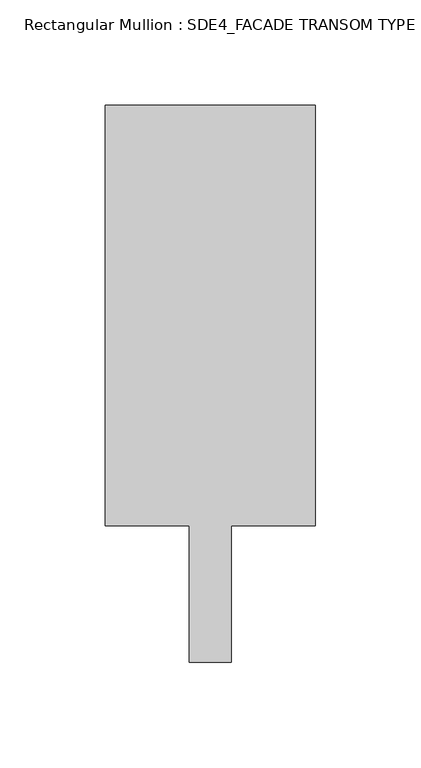
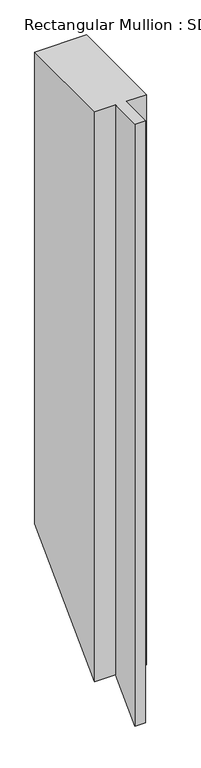
"""IFC4 building model written with IfcOpenShell, lengths in millimetres: member geometry, Rectangular Mullion : SDE4_FACADE TRANSOM TYPE 2."""

from ifc_helpers import new_model, si_unit, origin, place, context, project, spatial, faceted_brep, source, transform, mapped, element, save


def rectangular_mullion_sde4_facade_transom_type_2_6ebeb50c(model_context):
    return source(origin(), model_context, "Body", "Brep", [
        faceted_brep([(50.0, 132.5, 0.0), (-50.0, 132.5, 0.0), (-50.0, -67.5, 0.0), (-10.0, -67.5, 0.0), (-10.0, -132.5, 0.0), (10.0, -132.5, 0.0), (10.0, -67.5, 0.0), (50.0, -67.5, 0.0), (50.0, 132.5, -960.0), (-50.0, 132.5, -960.0), (-50.0, -67.5, -1160.0), (-10.0, -67.5, -1160.0), (-10.0, -132.5, -1225.0), (10.0, -132.5, -1225.0), (10.0, -67.5, -1160.0), (50.0, -67.5, -1160.0)], [[[0, 1, 2, 3, 4, 5, 6, 7]], [[1, 0, 8, 9]], [[2, 1, 9, 10]], [[3, 2, 10, 11]], [[4, 3, 11, 12]], [[5, 4, 12, 13]], [[6, 5, 13, 14]], [[7, 6, 14, 15]], [[0, 7, 15, 8]], [[8, 15, 14, 13, 12, 11, 10, 9]]]),
    ])


if __name__ == "__main__":
    model = new_model("IFC4")
    model_context = context("Model", 3, world=origin())
    ifc_project = project(units=[si_unit("LENGTHUNIT", "METRE", prefix="MILLI")], contexts=[model_context])
    site = spatial("IfcSite", under=ifc_project)
    building = spatial("IfcBuilding", under=site)
    placement = place(None, origin())
    rectangular_mullion_sde4_facade_transom_type_2_shape = rectangular_mullion_sde4_facade_transom_type_2_6ebeb50c(model_context)
    element("IfcMember", 1, ObjectType="Rectangular Mullion : SDE4_FACADE TRANSOM TYPE 2", at=placement, inside=building, context=model_context, shape_type="MappedRepresentation", body=[
        mapped(rectangular_mullion_sde4_facade_transom_type_2_shape, transform((0.0, 0.0, 0.0), x_axis=(1.0, 0.0, 0.0), y_axis=(0.0, 1.0, 0.0), z_axis=(0.0, 0.0, 1.0))),
    ])
    save(model, "model.ifc")

# Revit data of these elements
# Type "Rectangular Mullion : SDE4_FACADE TRANSOM TYPE 2"
#   built-in parameter 1007322 = 0.869423 (stored number, unit not read)
#   built-in parameter 1007321 = 0.164042 (stored number, unit not read)
#   built-in parameter 1007320 = 0.164042 (stored number, unit not read)
